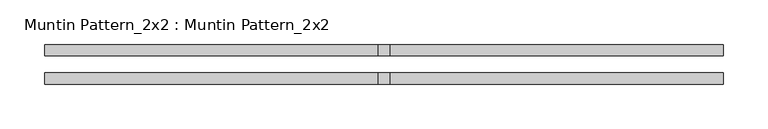
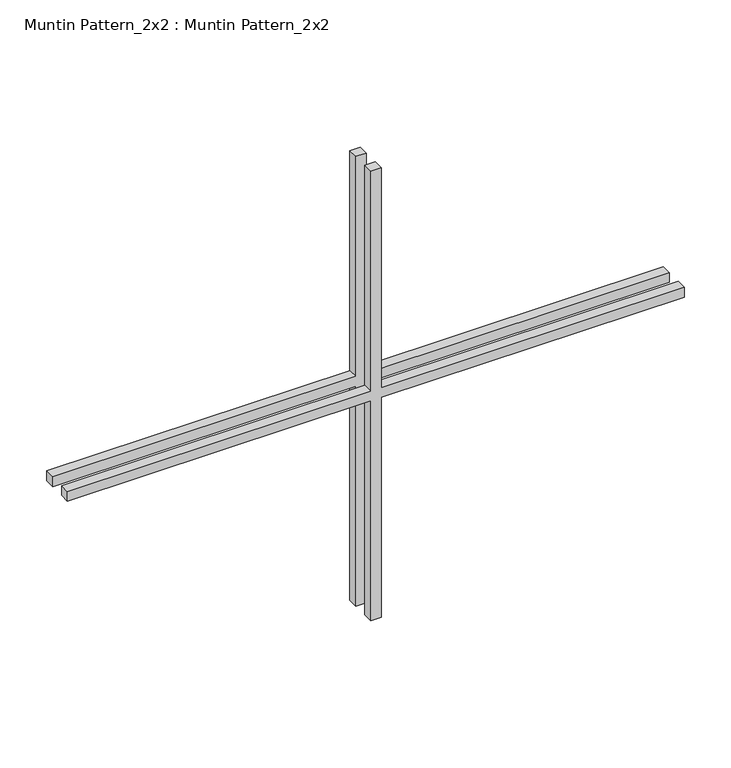
"""IFC4 building model written with IfcOpenShell, lengths in millimetres: proxy geometry, Muntin Pattern_2x2 : Muntin Pattern_2x2."""

from ifc_helpers import new_model, si_unit, frame, origin, place, context, project, spatial, polyline, outline, extrude, source, transform, mapped, element, save


def muntin_pattern_2x2_muntin_pattern_2x2_c1e6ccc8(model_context):
    return source(origin(), model_context, "Body", "SweptSolid", [
        extrude(outline(polyline([(300.0375, -6.35), (300.0375, -381.0), (287.3375, -381.0), (287.3375, -6.35), (0.0, -6.35), (0.0, 6.35), (287.3375, 6.35), (287.3375, 381.0), (300.0375, 381.0), (300.0375, 6.35), (587.375, 6.35), (587.375, -6.35), (300.0375, -6.35)])), frame((0.0, 9.525, 0.0), z_axis=(0.0, 1.0, 0.0), x_axis=(0.0, 0.0, 1.0)), (0.0, 0.0, 1.0), 12.7),
        extrude(outline(polyline([(300.0375, -6.35), (300.0375, -381.0), (287.3375, -381.0), (287.3375, -6.35), (0.0, -6.35), (0.0, 6.35), (287.3375, 6.35), (287.3375, 381.0), (300.0375, 381.0), (300.0375, 6.35), (587.375, 6.35), (587.375, -6.35), (300.0375, -6.35)])), frame((0.0, -22.225, 0.0), z_axis=(0.0, 1.0, 0.0), x_axis=(0.0, 0.0, 1.0)), (0.0, 0.0, 1.0), 12.7),
    ])


if __name__ == "__main__":
    model = new_model("IFC4")
    model_context = context("Model", 3, world=origin())
    ifc_project = project(units=[si_unit("LENGTHUNIT", "METRE", prefix="MILLI")], contexts=[model_context])
    site = spatial("IfcSite", under=ifc_project)
    building = spatial("IfcBuilding", under=site)
    placement = place(None, origin())
    muntin_pattern_2x2_muntin_pattern_2x2_shape = muntin_pattern_2x2_muntin_pattern_2x2_c1e6ccc8(model_context)
    element("IfcBuildingElementProxy", 1, Name="Muntin Pattern_2x2 : Muntin Pattern_2x2", ObjectType="Muntin Pattern_2x2 : Muntin Pattern_2x2", at=placement, inside=building, context=model_context, shape_type="MappedRepresentation", body=[
        mapped(muntin_pattern_2x2_muntin_pattern_2x2_shape, transform((0.0, 0.0, 0.0), x_axis=(1.0, 0.0, 0.0), y_axis=(0.0, 1.0, 0.0), z_axis=(0.0, 0.0, 1.0))),
    ])
    save(model, "model.ifc")

# Revit data of these elements
# Type "Muntin Pattern_2x2 : Muntin Pattern_2x2"
#   Width [instance default] = 4' - 0"
#   Thickness = 0' - 0 1/2"
#   Height [instance default] = 4' - 0"
#   Distance = 0' - 0 3/4"
#   Interior Material [instance default] = none
#   Exterior Material [instance default] = none
#   Default Elevation = 0
# Element 1 (IfcBuildingElementProxy, "Muntin Pattern_2x2 : Muntin Pattern_2x2")
#   Width = 2' - 6"
#   Height = 1' - 11 1/8"
#   Interior Material = Maple - Semigloss(Rotated)
#   Exterior Material = Clad - White
#   Materials on its faces: "Clad - White", "Maple - Semigloss(Rotated)"
# Materials
#   "Clad - White": class "Wood", colour RGB 245 245 243, transparency 0, Cost = 0
#   "Maple - Semigloss(Rotated)": class "Wood", colour RGB 196 161 118, transparency 0, Description = "Acer Saccharum", Cost = 0
